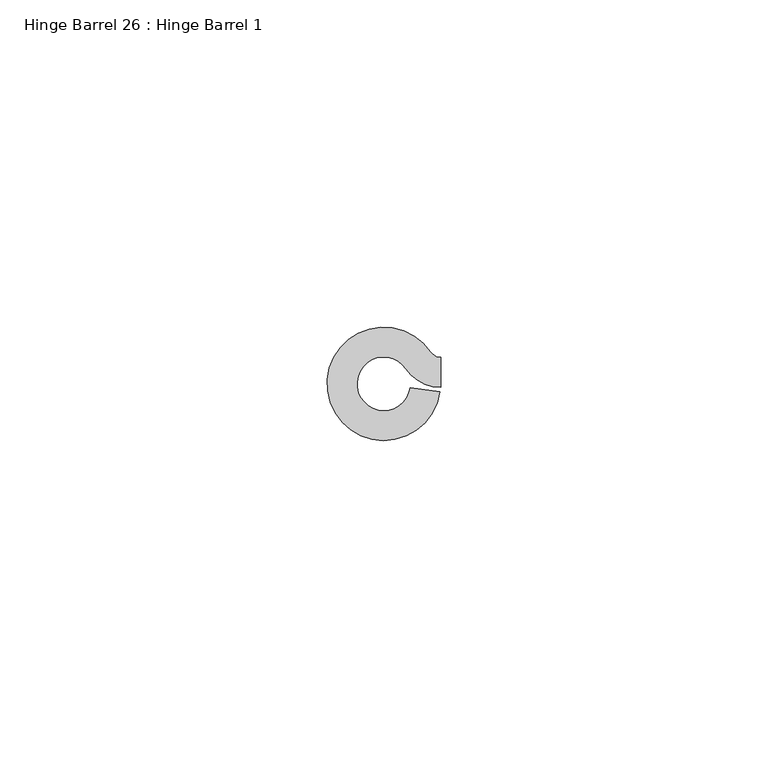
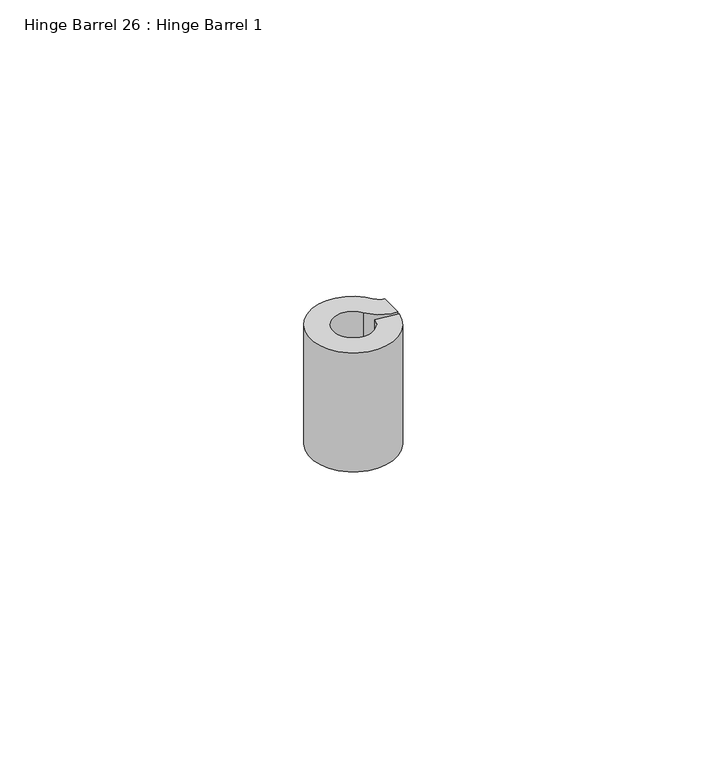
"""IFC4 building model written with IfcOpenShell, lengths in millimetres: proxy geometry, Hinge Barrel 26 : Hinge Barrel 1."""

import ifcopenshell
import ifcopenshell.guid

model = None  # the IFC model being written
_history = None  # IfcOwnerHistory: only IFC2X3 demands one
_inside = {}  # id of a spatial element -> (the spatial element, [elements in it])
_under = {}  # id of a project, library or spatial element -> (it, [spatial elements below it])
_declared = {}  # id of a project -> (the project, [libraries it declares])
_typed = {}  # id of a type object -> (the type object, [elements of that type])
_made_of = {}  # id of a material, layer set ... -> (it, [elements and type objects made of it])


def new_model(schema):
    """Start an empty IFC model of exactly this schema.

    Asked for "IFC4X3", IfcOpenShell would pick the latest addendum, in which some entities
    have other attributes; the version numbers below select the first issue.
    IFC2X3 requires an IfcOwnerHistory on every rooted entity: one is made here for all.
    """
    global model, _history
    if schema == "IFC4X3":
        model = ifcopenshell.file(schema_version=(4, 3, 0, 0))
    else:
        model = ifcopenshell.file(schema=schema)
    _inside.clear()
    _under.clear()
    _declared.clear()
    _typed.clear()
    _made_of.clear()
    _history = None
    if model.schema == "IFC2X3":
        org = make("IfcOrganization", Name="unknown")
        user = make(
            "IfcPersonAndOrganization",
            ThePerson=make("IfcPerson", FamilyName="unknown"),
            TheOrganization=org,
        )
        app = make(
            "IfcApplication",
            ApplicationDeveloper=org,
            Version="unknown",
            ApplicationFullName="unknown",
            ApplicationIdentifier="unknown",
        )
        _history = make(
            "IfcOwnerHistory",
            OwningUser=user,
            OwningApplication=app,
            ChangeAction="ADDED",
            CreationDate=0,
        )
    return model


def make(cls, **values):
    """One entity of the class cls with the attributes given. An attribute that is None is left unset."""
    return model.create_entity(
        cls, **{name: value for name, value in values.items() if value is not None}
    )


def rooted(cls, **values):
    """An entity with a GlobalId (a new one), such as an element, a storey or a relation."""
    return make(cls, GlobalId=ifcopenshell.guid.new(), OwnerHistory=_history, **values)


def si_unit(unit_type, name, prefix=None):
    """IfcSIUnit, for example si_unit("LENGTHUNIT", "METRE", prefix="MILLI")."""
    return make("IfcSIUnit", UnitType=unit_type, Prefix=prefix, Name=name)


def assignment(units):
    """IfcUnitAssignment: the units of a project."""
    return None if units is None else make("IfcUnitAssignment", Units=units)


def point(xyz):
    """IfcCartesianPoint."""
    return None if xyz is None else make("IfcCartesianPoint", Coordinates=xyz)


def direction(xyz):
    """IfcDirection."""
    return None if xyz is None else make("IfcDirection", DirectionRatios=xyz)


def frame(location, z_axis=None, x_axis=None):
    """IfcAxis2Placement3D, a coordinate frame: its origin and axes. An axis left out is left unset."""
    return make(
        "IfcAxis2Placement3D",
        Location=point(location),
        Axis=direction(z_axis),
        RefDirection=direction(x_axis),
    )


def frame_2d(location, x_axis=None):
    """IfcAxis2Placement2D, a coordinate frame in the plane: its origin and x axis."""
    return make(
        "IfcAxis2Placement2D", Location=point(location), RefDirection=direction(x_axis)
    )


def origin():
    """The frame at (0, 0, 0) with its axes left unset."""
    return frame((0.0, 0.0, 0.0))


def place(relative_to, where):
    """IfcLocalPlacement: puts the frame where relative to a parent placement (None: the world)."""
    return make(
        "IfcLocalPlacement", PlacementRelTo=relative_to, RelativePlacement=where
    )


def context(
    kind, dimensions, precision=None, world=None, true_north=None, identifier=None
):
    """IfcGeometricRepresentationContext, for example the 3D "Model" context."""
    return make(
        "IfcGeometricRepresentationContext",
        ContextIdentifier=identifier,
        ContextType=kind,
        CoordinateSpaceDimension=dimensions,
        Precision=precision,
        WorldCoordinateSystem=world,
        TrueNorth=true_north,
    )


def project(units=None, contexts=None):
    """IfcProject with its units and contexts."""
    return rooted(
        "IfcProject",
        Name="project",
        RepresentationContexts=contexts,
        UnitsInContext=assignment(units),
    )


def spatial(cls, under=None, at=None, **own):
    """A site, building, storey or space (cls), placed at a placement, below another one or the project."""
    s = rooted(cls, ObjectPlacement=at, **own)
    if under is not None:
        _under.setdefault(under.id(), (under, []))[1].append(s)
    return s


def polyline(points):
    """IfcPolyline through the points."""
    return make("IfcPolyline", Points=[point(p) for p in points])


def circle_curve(where, radius):
    """IfcCircle in the frame where."""
    return make("IfcCircle", Position=where, Radius=radius)


def trimmed(basis, trim1, trim2, sense, master):
    """IfcTrimmedCurve: the piece of a basis curve between two trims."""
    return make(
        "IfcTrimmedCurve",
        BasisCurve=basis,
        Trim1=trim1,
        Trim2=trim2,
        SenseAgreement=sense,
        MasterRepresentation=master,
    )


def segment(curve, same_sense, transition):
    """IfcCompositeCurveSegment."""
    return make(
        "IfcCompositeCurveSegment",
        Transition=transition,
        SameSense=same_sense,
        ParentCurve=curve,
    )


def composite_curve(segments, self_intersect=None):
    """IfcCompositeCurve: segments joined end to end."""
    return make("IfcCompositeCurve", Segments=segments, SelfIntersect=self_intersect)


def outline(outer, holes=None, kind="AREA"):
    """IfcArbitraryClosedProfileDef: a profile drawn as a closed curve; with holes, ...WithVoids."""
    if holes is None:
        return make("IfcArbitraryClosedProfileDef", ProfileType=kind, OuterCurve=outer)
    return make(
        "IfcArbitraryProfileDefWithVoids",
        ProfileType=kind,
        OuterCurve=outer,
        InnerCurves=holes,
    )


def extrude(swept, where, along, depth):
    """IfcExtrudedAreaSolid: the profile swept, set in the frame where, extruded along a direction by depth."""
    return make(
        "IfcExtrudedAreaSolid",
        SweptArea=swept,
        Position=where,
        ExtrudedDirection=direction(along),
        Depth=depth,
    )


def shape(context_of_items, identifier, shape_type, items):
    """IfcShapeRepresentation: the items that make up one representation, for example the "Body"."""
    return make(
        "IfcShapeRepresentation",
        ContextOfItems=context_of_items,
        RepresentationIdentifier=identifier,
        RepresentationType=shape_type,
        Items=items,
    )


def source(mapping_origin, context_of_items, identifier, shape_type, items):
    """IfcRepresentationMap: a shape defined once, which mapped items show again and again."""
    return make(
        "IfcRepresentationMap",
        MappingOrigin=mapping_origin,
        MappedRepresentation=shape(context_of_items, identifier, shape_type, items),
    )


def transform(
    local_origin,
    x_axis=None,
    y_axis=None,
    z_axis=None,
    scale=None,
    scale2=None,
    scale3=None,
    uniform=True,
):
    """IfcCartesianTransformationOperator3D, or its non-uniform kind. x_axis, y_axis, z_axis: its Axis1, 2, 3."""
    if uniform:
        return make(
            "IfcCartesianTransformationOperator3D",
            Axis1=direction(x_axis),
            Axis2=direction(y_axis),
            LocalOrigin=point(local_origin),
            Scale=scale,
            Axis3=direction(z_axis),
        )
    return make(
        "IfcCartesianTransformationOperator3DnonUniform",
        Axis1=direction(x_axis),
        Axis2=direction(y_axis),
        LocalOrigin=point(local_origin),
        Scale=scale,
        Axis3=direction(z_axis),
        Scale2=scale2,
        Scale3=scale3,
    )


def mapped(mapping_source, mapping_target):
    """IfcMappedItem: shows the shape of a source again, moved by a transform."""
    return make(
        "IfcMappedItem", MappingSource=mapping_source, MappingTarget=mapping_target
    )


def made_of(thing, what):
    """Note that an element or type object is made of a material, layer set ...; save() writes the relation."""
    if what is not None:
        _made_of.setdefault(what.id(), (what, []))[1].append(thing)
    return thing


def element(
    cls,
    number,
    at=None,
    inside=None,
    cuts=None,
    type_object=None,
    material=None,
    context=None,
    identifier="Body",
    shape_type=None,
    held_by="IfcProductDefinitionShape",
    body=None,
    shapes=None,
    **own,
):
    """One element of the class cls, such as IfcWall. Its Tag is "e" and its number.

    at: its placement. inside: the storey or other place that contains it. cuts: it is an
    opening in that element (IfcRelVoidsElement). A single representation is given by context,
    identifier, shape_type and body (its items); several are given by shapes. held_by: the class
    of the entity that holds the representations. save() writes the other relations.
    """
    e = rooted(cls, Tag="e%d" % number, ObjectPlacement=at, **own)
    if body is not None:
        shapes = [shape(context, identifier, shape_type, body)]
    if shapes is not None:
        e.Representation = make(held_by, Representations=shapes)
    if inside is not None:
        _inside.setdefault(inside.id(), (inside, []))[1].append(e)
    if cuts is not None:
        rooted(
            "IfcRelVoidsElement", RelatingBuildingElement=cuts, RelatedOpeningElement=e
        )
    if type_object is not None:
        _typed.setdefault(type_object.id(), (type_object, []))[1].append(e)
    return made_of(e, material)


def aggregate(whole, parts):
    """IfcRelAggregates: a whole, such as a stair, and the parts it consists of."""
    return rooted("IfcRelAggregates", RelatingObject=whole, RelatedObjects=parts)


def save(model, path):
    """Write the relations noted so far, then the file.

    IfcRelAggregates (storeys below a building ...), IfcRelContainedInSpatialStructure (elements
    in a storey), IfcRelDefinesByType, IfcRelAssociatesMaterial and IfcRelDeclares: one each for
    every whole, place, type object, material and project.
    """
    for whole, parts in _under.values():
        aggregate(whole, parts)
    for where, things in _inside.values():
        rooted(
            "IfcRelContainedInSpatialStructure",
            RelatedElements=things,
            RelatingStructure=where,
        )
    for kind, things in _typed.values():
        rooted("IfcRelDefinesByType", RelatedObjects=things, RelatingType=kind)
    for what, things in _made_of.values():
        rooted("IfcRelAssociatesMaterial", RelatedObjects=things, RelatingMaterial=what)
    for by, libraries in _declared.values():
        rooted("IfcRelDeclares", RelatingContext=by, RelatedDefinitions=libraries)
    model.write(path)


def hinge_barrel_26_hinge_barrel_1_b61994a4(model_context):
    return source(origin(), model_context, "Body", "SweptSolid", [
        extrude(outline(composite_curve([segment(trimmed(circle_curve(frame_2d((587319.1320739, -531776.6049841)), 4.0894), [point((587322.5194669, -531774.3139665))], [point((587323.1821338, -531777.1708529))], True, "CARTESIAN"), True, "CONTINUOUS"), segment(polyline([(587323.1821338, -531777.1708529), (587327.7022899, -531777.8024028)]), True, "CONTINUOUS"), segment(trimmed(circle_curve(frame_2d((587319.1320739, -531776.6049841)), 8.6534625), [point((587327.7022899, -531777.8024028))], [point((587326.3000393, -531771.7570273))], False, "CARTESIAN"), True, "CONTINUOUS"), segment(trimmed(circle_curve(frame_2d((587327.8245257, -531770.7259615)), 1.8404226), [point((587326.3000393, -531771.7570273))], [point((587327.8245257, -531772.5663841))], True, "CARTESIAN"), True, "CONTINUOUS"), segment(polyline([(587327.8245257, -531772.5663841), (587327.8245257, -531777.1304466)]), True, "CONTINUOUS"), segment(trimmed(circle_curve(frame_2d((587327.8245257, -531770.7259615)), 6.4044851), [point((587327.8245257, -531777.1304466))], [point((587322.5194669, -531774.3139665))], False, "CARTESIAN"), True, "CONTINUOUS")], self_intersect=False)), frame((0.0, 0.0, 1149.35), z_axis=(0.0, 0.0, 1.0), x_axis=(1.0, 0.0, 0.0)), (0.0, 0.0, 1.0), 25.4),
    ])


if __name__ == "__main__":
    model = new_model("IFC4")
    model_context = context("Model", 3, world=origin())
    ifc_project = project(units=[si_unit("LENGTHUNIT", "METRE", prefix="MILLI")], contexts=[model_context])
    site = spatial("IfcSite", under=ifc_project)
    building = spatial("IfcBuilding", under=site)
    placement = place(None, origin())
    hinge_barrel_26_hinge_barrel_1_shape = hinge_barrel_26_hinge_barrel_1_b61994a4(model_context)
    element("IfcBuildingElementProxy", 1, Name="Hinge Barrel 26 : Hinge Barrel 1", ObjectType="Hinge Barrel 26 : Hinge Barrel 1", at=placement, inside=building, context=model_context, shape_type="MappedRepresentation", body=[
        mapped(hinge_barrel_26_hinge_barrel_1_shape, transform((0.0, 0.0, 0.0), x_axis=(1.0, 0.0, 0.0), y_axis=(0.0, 1.0, 0.0), z_axis=(0.0, 0.0, 1.0))),
    ])
    save(model, "model.ifc")

# Revit data of these elements
# Element 1 (IfcBuildingElementProxy, "Hinge Barrel 26 : Hinge Barrel 1")
#   Materials on its faces: "6\"X6\" WELD-ON STL BUTT HINGE"
# Materials
#   "6\"X6\" WELD-ON STL BUTT HINGE": class "Metal", colour RGB 189 187 185, transparency 0, Description = "Carbon steel", Cost = 0
